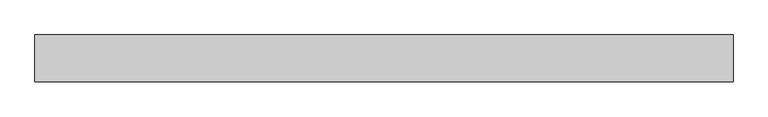
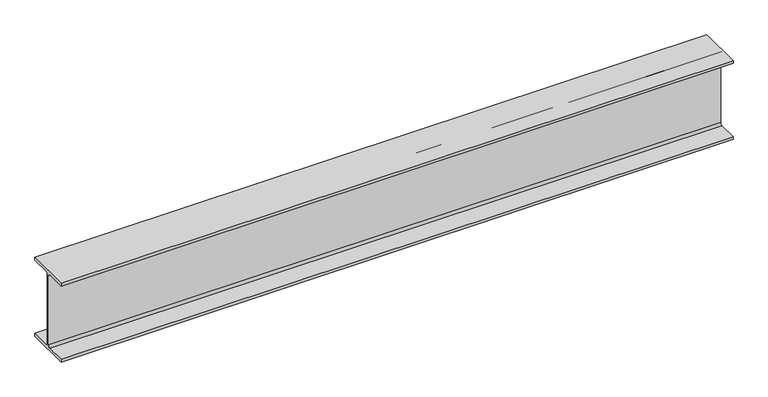
"""IFC4 building model written with IfcOpenShell, lengths in millimetres: beam geometry, Steel Beam_H-KSD3502 : H_SB_ASB_H-194x150x6x9."""

import ifcopenshell
import ifcopenshell.guid

model = None  # the IFC model being written
_history = None  # IfcOwnerHistory: only IFC2X3 demands one
_inside = {}  # id of a spatial element -> (the spatial element, [elements in it])
_under = {}  # id of a project, library or spatial element -> (it, [spatial elements below it])
_declared = {}  # id of a project -> (the project, [libraries it declares])
_typed = {}  # id of a type object -> (the type object, [elements of that type])
_made_of = {}  # id of a material, layer set ... -> (it, [elements and type objects made of it])


def new_model(schema):
    """Start an empty IFC model of exactly this schema.

    Asked for "IFC4X3", IfcOpenShell would pick the latest addendum, in which some entities
    have other attributes; the version numbers below select the first issue.
    IFC2X3 requires an IfcOwnerHistory on every rooted entity: one is made here for all.
    """
    global model, _history
    if schema == "IFC4X3":
        model = ifcopenshell.file(schema_version=(4, 3, 0, 0))
    else:
        model = ifcopenshell.file(schema=schema)
    _inside.clear()
    _under.clear()
    _declared.clear()
    _typed.clear()
    _made_of.clear()
    _history = None
    if model.schema == "IFC2X3":
        org = make("IfcOrganization", Name="unknown")
        user = make(
            "IfcPersonAndOrganization",
            ThePerson=make("IfcPerson", FamilyName="unknown"),
            TheOrganization=org,
        )
        app = make(
            "IfcApplication",
            ApplicationDeveloper=org,
            Version="unknown",
            ApplicationFullName="unknown",
            ApplicationIdentifier="unknown",
        )
        _history = make(
            "IfcOwnerHistory",
            OwningUser=user,
            OwningApplication=app,
            ChangeAction="ADDED",
            CreationDate=0,
        )
    return model


def make(cls, **values):
    """One entity of the class cls with the attributes given. An attribute that is None is left unset."""
    return model.create_entity(
        cls, **{name: value for name, value in values.items() if value is not None}
    )


def rooted(cls, **values):
    """An entity with a GlobalId (a new one), such as an element, a storey or a relation."""
    return make(cls, GlobalId=ifcopenshell.guid.new(), OwnerHistory=_history, **values)


def si_unit(unit_type, name, prefix=None):
    """IfcSIUnit, for example si_unit("LENGTHUNIT", "METRE", prefix="MILLI")."""
    return make("IfcSIUnit", UnitType=unit_type, Prefix=prefix, Name=name)


def assignment(units):
    """IfcUnitAssignment: the units of a project."""
    return None if units is None else make("IfcUnitAssignment", Units=units)


def point(xyz):
    """IfcCartesianPoint."""
    return None if xyz is None else make("IfcCartesianPoint", Coordinates=xyz)


def direction(xyz):
    """IfcDirection."""
    return None if xyz is None else make("IfcDirection", DirectionRatios=xyz)


def frame(location, z_axis=None, x_axis=None):
    """IfcAxis2Placement3D, a coordinate frame: its origin and axes. An axis left out is left unset."""
    return make(
        "IfcAxis2Placement3D",
        Location=point(location),
        Axis=direction(z_axis),
        RefDirection=direction(x_axis),
    )


def frame_2d(location, x_axis=None):
    """IfcAxis2Placement2D, a coordinate frame in the plane: its origin and x axis."""
    return make(
        "IfcAxis2Placement2D", Location=point(location), RefDirection=direction(x_axis)
    )


def origin():
    """The frame at (0, 0, 0) with its axes left unset."""
    return frame((0.0, 0.0, 0.0))


def place(relative_to, where):
    """IfcLocalPlacement: puts the frame where relative to a parent placement (None: the world)."""
    return make(
        "IfcLocalPlacement", PlacementRelTo=relative_to, RelativePlacement=where
    )


def context(
    kind, dimensions, precision=None, world=None, true_north=None, identifier=None
):
    """IfcGeometricRepresentationContext, for example the 3D "Model" context."""
    return make(
        "IfcGeometricRepresentationContext",
        ContextIdentifier=identifier,
        ContextType=kind,
        CoordinateSpaceDimension=dimensions,
        Precision=precision,
        WorldCoordinateSystem=world,
        TrueNorth=true_north,
    )


def project(units=None, contexts=None):
    """IfcProject with its units and contexts."""
    return rooted(
        "IfcProject",
        Name="project",
        RepresentationContexts=contexts,
        UnitsInContext=assignment(units),
    )


def spatial(cls, under=None, at=None, **own):
    """A site, building, storey or space (cls), placed at a placement, below another one or the project."""
    s = rooted(cls, ObjectPlacement=at, **own)
    if under is not None:
        _under.setdefault(under.id(), (under, []))[1].append(s)
    return s


def polyline(points):
    """IfcPolyline through the points."""
    return make("IfcPolyline", Points=[point(p) for p in points])


def circle_curve(where, radius):
    """IfcCircle in the frame where."""
    return make("IfcCircle", Position=where, Radius=radius)


def trimmed(basis, trim1, trim2, sense, master):
    """IfcTrimmedCurve: the piece of a basis curve between two trims."""
    return make(
        "IfcTrimmedCurve",
        BasisCurve=basis,
        Trim1=trim1,
        Trim2=trim2,
        SenseAgreement=sense,
        MasterRepresentation=master,
    )


def segment(curve, same_sense, transition):
    """IfcCompositeCurveSegment."""
    return make(
        "IfcCompositeCurveSegment",
        Transition=transition,
        SameSense=same_sense,
        ParentCurve=curve,
    )


def composite_curve(segments, self_intersect=None):
    """IfcCompositeCurve: segments joined end to end."""
    return make("IfcCompositeCurve", Segments=segments, SelfIntersect=self_intersect)


def outline(outer, holes=None, kind="AREA"):
    """IfcArbitraryClosedProfileDef: a profile drawn as a closed curve; with holes, ...WithVoids."""
    if holes is None:
        return make("IfcArbitraryClosedProfileDef", ProfileType=kind, OuterCurve=outer)
    return make(
        "IfcArbitraryProfileDefWithVoids",
        ProfileType=kind,
        OuterCurve=outer,
        InnerCurves=holes,
    )


def extrude(swept, where, along, depth):
    """IfcExtrudedAreaSolid: the profile swept, set in the frame where, extruded along a direction by depth."""
    return make(
        "IfcExtrudedAreaSolid",
        SweptArea=swept,
        Position=where,
        ExtrudedDirection=direction(along),
        Depth=depth,
    )


def shape(context_of_items, identifier, shape_type, items):
    """IfcShapeRepresentation: the items that make up one representation, for example the "Body"."""
    return make(
        "IfcShapeRepresentation",
        ContextOfItems=context_of_items,
        RepresentationIdentifier=identifier,
        RepresentationType=shape_type,
        Items=items,
    )


def source(mapping_origin, context_of_items, identifier, shape_type, items):
    """IfcRepresentationMap: a shape defined once, which mapped items show again and again."""
    return make(
        "IfcRepresentationMap",
        MappingOrigin=mapping_origin,
        MappedRepresentation=shape(context_of_items, identifier, shape_type, items),
    )


def transform(
    local_origin,
    x_axis=None,
    y_axis=None,
    z_axis=None,
    scale=None,
    scale2=None,
    scale3=None,
    uniform=True,
):
    """IfcCartesianTransformationOperator3D, or its non-uniform kind. x_axis, y_axis, z_axis: its Axis1, 2, 3."""
    if uniform:
        return make(
            "IfcCartesianTransformationOperator3D",
            Axis1=direction(x_axis),
            Axis2=direction(y_axis),
            LocalOrigin=point(local_origin),
            Scale=scale,
            Axis3=direction(z_axis),
        )
    return make(
        "IfcCartesianTransformationOperator3DnonUniform",
        Axis1=direction(x_axis),
        Axis2=direction(y_axis),
        LocalOrigin=point(local_origin),
        Scale=scale,
        Axis3=direction(z_axis),
        Scale2=scale2,
        Scale3=scale3,
    )


def mapped(mapping_source, mapping_target):
    """IfcMappedItem: shows the shape of a source again, moved by a transform."""
    return make(
        "IfcMappedItem", MappingSource=mapping_source, MappingTarget=mapping_target
    )


def made_of(thing, what):
    """Note that an element or type object is made of a material, layer set ...; save() writes the relation."""
    if what is not None:
        _made_of.setdefault(what.id(), (what, []))[1].append(thing)
    return thing


def element(
    cls,
    number,
    at=None,
    inside=None,
    cuts=None,
    type_object=None,
    material=None,
    context=None,
    identifier="Body",
    shape_type=None,
    held_by="IfcProductDefinitionShape",
    body=None,
    shapes=None,
    **own,
):
    """One element of the class cls, such as IfcWall. Its Tag is "e" and its number.

    at: its placement. inside: the storey or other place that contains it. cuts: it is an
    opening in that element (IfcRelVoidsElement). A single representation is given by context,
    identifier, shape_type and body (its items); several are given by shapes. held_by: the class
    of the entity that holds the representations. save() writes the other relations.
    """
    e = rooted(cls, Tag="e%d" % number, ObjectPlacement=at, **own)
    if body is not None:
        shapes = [shape(context, identifier, shape_type, body)]
    if shapes is not None:
        e.Representation = make(held_by, Representations=shapes)
    if inside is not None:
        _inside.setdefault(inside.id(), (inside, []))[1].append(e)
    if cuts is not None:
        rooted(
            "IfcRelVoidsElement", RelatingBuildingElement=cuts, RelatedOpeningElement=e
        )
    if type_object is not None:
        _typed.setdefault(type_object.id(), (type_object, []))[1].append(e)
    return made_of(e, material)


def aggregate(whole, parts):
    """IfcRelAggregates: a whole, such as a stair, and the parts it consists of."""
    return rooted("IfcRelAggregates", RelatingObject=whole, RelatedObjects=parts)


def save(model, path):
    """Write the relations noted so far, then the file.

    IfcRelAggregates (storeys below a building ...), IfcRelContainedInSpatialStructure (elements
    in a storey), IfcRelDefinesByType, IfcRelAssociatesMaterial and IfcRelDeclares: one each for
    every whole, place, type object, material and project.
    """
    for whole, parts in _under.values():
        aggregate(whole, parts)
    for where, things in _inside.values():
        rooted(
            "IfcRelContainedInSpatialStructure",
            RelatedElements=things,
            RelatingStructure=where,
        )
    for kind, things in _typed.values():
        rooted("IfcRelDefinesByType", RelatedObjects=things, RelatingType=kind)
    for what, things in _made_of.values():
        rooted("IfcRelAssociatesMaterial", RelatedObjects=things, RelatingMaterial=what)
    for by, libraries in _declared.values():
        rooted("IfcRelDeclares", RelatingContext=by, RelatedDefinitions=libraries)
    model.write(path)


def beam_59e108a4(model_context):
    return source(origin(), model_context, "Body", "SweptSolid", [
        extrude(outline(composite_curve([segment(polyline([(82.5, -141.5), (82.5, -151.7), (-82.5, -151.7), (-82.5, -141.5), (-11.9, -141.5)]), True, "CONTINUOUS"), segment(trimmed(circle_curve(frame_2d((-11.9, -132.6)), 8.9), [point((-11.9, -141.5))], [point((-3.0, -132.6))], True, "CARTESIAN"), True, "CONTINUOUS"), segment(polyline([(-3.0, -132.6), (-3.0, 132.6)]), True, "CONTINUOUS"), segment(trimmed(circle_curve(frame_2d((-11.9, 132.6)), 8.9), [point((-3.0, 132.6))], [point((-11.9, 141.5))], True, "CARTESIAN"), True, "CONTINUOUS"), segment(polyline([(-11.9, 141.5), (-82.5, 141.5), (-82.5, 151.7), (82.5, 151.7), (82.5, 141.5), (11.9, 141.5)]), True, "CONTINUOUS"), segment(trimmed(circle_curve(frame_2d((11.9, 132.6)), 8.9), [point((11.9, 141.5))], [point((3.0, 132.6))], True, "CARTESIAN"), True, "CONTINUOUS"), segment(polyline([(3.0, 132.6), (3.0, -132.6)]), True, "CONTINUOUS"), segment(trimmed(circle_curve(frame_2d((11.9, -132.6)), 8.9), [point((3.0, -132.6))], [point((11.9, -141.5))], True, "CARTESIAN"), True, "CONTINUOUS"), segment(polyline([(11.9, -141.5), (82.5, -141.5)]), True, "CONTINUOUS")], self_intersect=False)), frame((-1200.0, 0.0, 0.0), z_axis=(1.0, 0.0, 0.0), x_axis=(0.0, 1.0, 0.0)), (0.0, 0.0, 1.0), 2453.1701073),
    ])


if __name__ == "__main__":
    model = new_model("IFC4")
    model_context = context("Model", 3, world=origin())
    ifc_project = project(units=[si_unit("LENGTHUNIT", "METRE", prefix="MILLI")], contexts=[model_context])
    site = spatial("IfcSite", under=ifc_project)
    building = spatial("IfcBuilding", under=site)
    placement = place(None, origin())
    beam_shape = beam_59e108a4(model_context)
    element("IfcBeam", 1, ObjectType="Steel Beam_H-KSD3502 : H_SB_ASB_H-194x150x6x9", at=placement, inside=building, context=model_context, shape_type="MappedRepresentation", body=[
        mapped(beam_shape, transform((0.0, 0.0, 0.0), x_axis=(1.0, 0.0, 0.0), y_axis=(0.0, 1.0, 0.0), z_axis=(0.0, 0.0, 1.0))),
    ])
    save(model, "model.ifc")

# Revit data of these elements
# Type "Steel Beam_H-KSD3502 : H_SB_ASB_H-194x150x6x9"
#   Width = 15.0 cm
#   Web Thickness = 0.6 cm
#   Web Fillet = 1.3 cm
#   Warping Constant = 43316.0 cm⁶
#   Torsional Moment of Inertia = 8.622 cm⁴
#   Torsional Modulus = 1.0 cm³
#   Section Area = 39.01 cm²
#   Plastic Modulus weak axis = 104.0 cm³
#   Plastic Modulus strong axis = 309.0 cm³
#   Perimeter = 0.95 m²/m
#   Nominal Weight = 30.60 kgf/m
#   Moment of Inertia weak axis = 507.00 cm⁴
#   Moment of Inertia strong axis = 2690.00 cm⁴
#   Height = 19.4 cm
#   Flange Thickness = 0.9 cm
#   Elastic Modulus weak axis = 67.6 cm³
#   Elastic Modulus strong axis = 277.0 cm³
#   Centroid Vertical = 9.7 cm
#   Centroid Horizontal = 7.5 cm
#   Length [instance default] = 1.5240 m
#   Structural Material [instance default] = Steel, 45-345
#   Assembly Code = ""
# Element 1 (IfcBeam, "Steel Beam_H-KSD3502 : H_SB_ASB_H-194x150x6x9")
#   Structural Material = none
# Materials
#   "Steel, 45-345": class "Metal", colour RGB 189 187 185, transparency 0, Description = "Steel 345 MPa", Cost = 0
